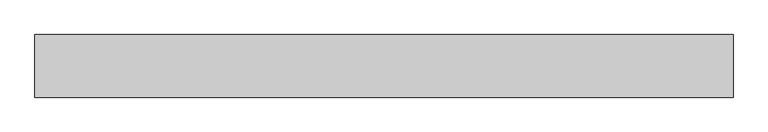
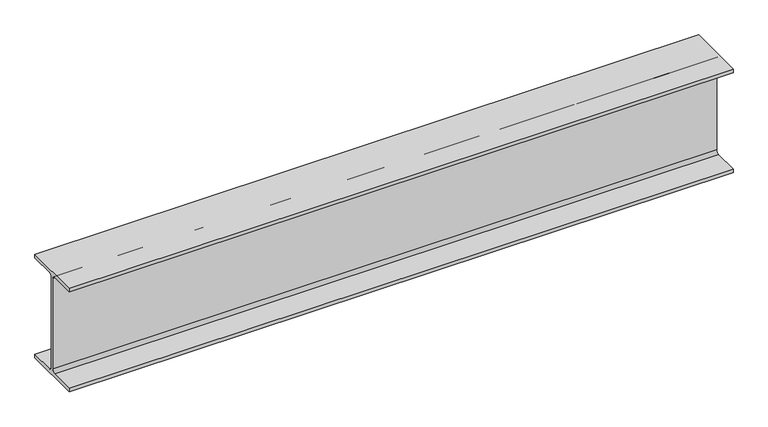
"""IFC4 building model written with IfcOpenShell, lengths in millimetres: beam geometry, Old_Steel Beam_H-KSD3502 : H_SB_ASB_H-194×150x6x9."""

from ifc_helpers import new_model, si_unit, point, frame, frame_2d, origin, place, context, project, spatial, polyline, circle_curve, trimmed, segment, composite_curve, outline, extrude, source, transform, mapped, element, save


def beam_885278b6(model_context):
    return source(origin(), model_context, "Body", "SweptSolid", [
        extrude(outline(composite_curve([segment(polyline([(82.5, -141.5), (82.5, -151.7), (-82.5, -151.7), (-82.5, -141.5), (-11.9, -141.5)]), True, "CONTINUOUS"), segment(trimmed(circle_curve(frame_2d((-11.9, -132.6)), 8.9), [point((-11.9, -141.5))], [point((-3.0, -132.6))], True, "CARTESIAN"), True, "CONTINUOUS"), segment(polyline([(-3.0, -132.6), (-3.0, 132.6)]), True, "CONTINUOUS"), segment(trimmed(circle_curve(frame_2d((-11.9, 132.6)), 8.9), [point((-3.0, 132.6))], [point((-11.9, 141.5))], True, "CARTESIAN"), True, "CONTINUOUS"), segment(polyline([(-11.9, 141.5), (-82.5, 141.5), (-82.5, 151.7), (82.5, 151.7), (82.5, 141.5), (11.9, 141.5)]), True, "CONTINUOUS"), segment(trimmed(circle_curve(frame_2d((11.9, 132.6)), 8.9), [point((11.9, 141.5))], [point((3.0, 132.6))], True, "CARTESIAN"), True, "CONTINUOUS"), segment(polyline([(3.0, 132.6), (3.0, -132.6)]), True, "CONTINUOUS"), segment(trimmed(circle_curve(frame_2d((11.9, -132.6)), 8.9), [point((3.0, -132.6))], [point((11.9, -141.5))], True, "CARTESIAN"), True, "CONTINUOUS"), segment(polyline([(11.9, -141.5), (82.5, -141.5)]), True, "CONTINUOUS")], self_intersect=False)), frame((-851.3274068, 0.0, 0.0), z_axis=(1.0, 0.0, 0.0), x_axis=(0.0, 1.0, 0.0)), (0.0, 0.0, 1.0), 1839.6820153),
    ])


if __name__ == "__main__":
    model = new_model("IFC4")
    model_context = context("Model", 3, world=origin())
    ifc_project = project(units=[si_unit("LENGTHUNIT", "METRE", prefix="MILLI")], contexts=[model_context])
    site = spatial("IfcSite", under=ifc_project)
    building = spatial("IfcBuilding", under=site)
    placement = place(None, origin())
    beam_shape = beam_885278b6(model_context)
    element("IfcBeam", 1, ObjectType="Old_Steel Beam_H-KSD3502 : H_SB_ASB_H-194×150x6x9", at=placement, inside=building, context=model_context, shape_type="MappedRepresentation", body=[
        mapped(beam_shape, transform((0.0, 0.0, 0.0), x_axis=(1.0, 0.0, 0.0), y_axis=(0.0, 1.0, 0.0), z_axis=(0.0, 0.0, 1.0))),
    ])
    save(model, "model.ifc")

# Revit data of these elements
# Type "Old_Steel Beam_H-KSD3502 : H_SB_ASB_H-194×150x6x9"
#   Width = 15.0 cm
#   Web Thickness = 0.6 cm
#   Web Fillet = 1.3 cm
#   Warping Constant = 43316.0 cm⁶
#   Torsional Moment of Inertia = 8.622 cm⁴
#   Torsional Modulus = 1.0 cm³
#   Section Area = 39.01 cm²
#   Plastic Modulus weak axis = 104.0 cm³
#   Plastic Modulus strong axis = 309.0 cm³
#   Perimeter = 0.95 m²/m
#   Nominal Weight = 30.60 kgf/m
#   Moment of Inertia weak axis = 507.00 cm⁴
#   Moment of Inertia strong axis = 2690.00 cm⁴
#   Height = 19.4 cm
#   Flange Thickness = 0.9 cm
#   Elastic Modulus weak axis = 67.6 cm³
#   Elastic Modulus strong axis = 277.0 cm³
#   Centroid Vertical = 9.7 cm
#   Centroid Horizontal = 7.5 cm
#   Length [instance default] = 1.5240 m
#   Structural Material [instance default] = Steel, 45-345
#   Assembly Code = ""
# Element 1 (IfcBeam, "Old_Steel Beam_H-KSD3502 : H_SB_ASB_H-194×150x6x9")
#   Structural Material = none
# Materials
#   "Steel, 45-345": class "Metal", colour RGB 189 187 185, transparency 0, Description = "Steel 345 MPa", Cost = 0
